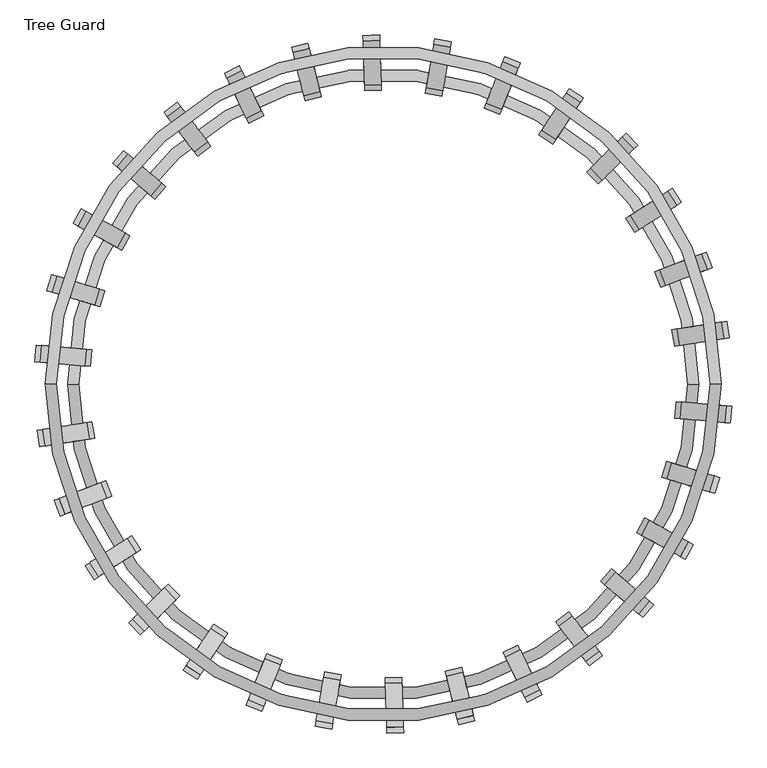
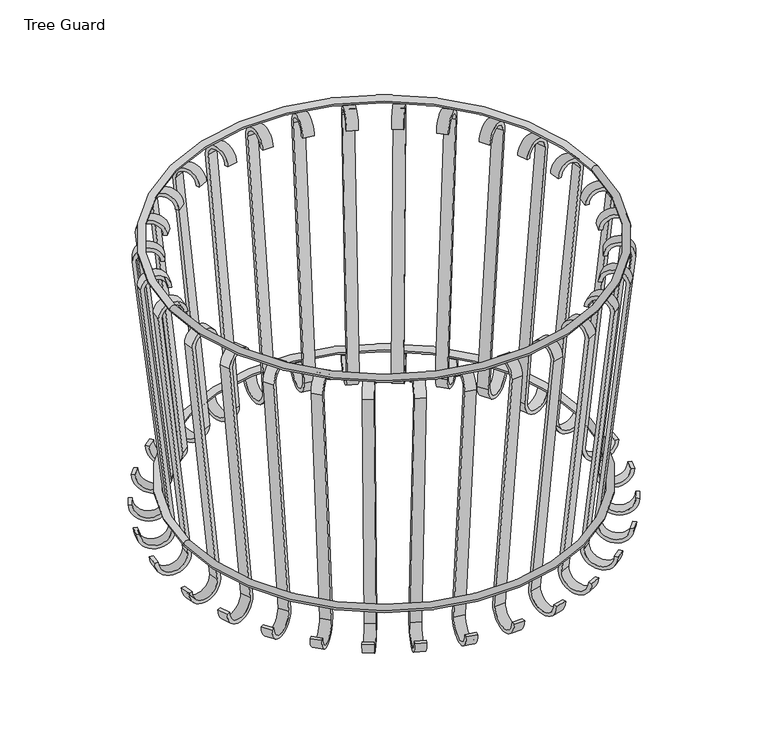
"""IFC4 building model written with IfcOpenShell, lengths in millimetres: railing geometry, Tree Guard."""

from ifc_helpers import new_model, si_unit, point, frame, frame_2d, origin, origin_2d, place, context, project, spatial, polyline, circle_curve, ellipse_curve, trimmed, segment, composite_curve, outline, extrude, source, transform, mapped, element, save
from ifc_brep_helpers import revolved_surface, advanced_brep


def tree_guard_4b5819f2(model_context):
    return source(origin(), model_context, "Body", "SolidModel", [
        advanced_brep(
        [(1686.3981957, 17584.520735, 1003.3), (3235.7981957, 17584.520735, 1003.3), (3210.3981957, 17584.520735, 1003.3), (1711.7981957, 17584.520735, 1003.3)],
        [
            (0, 1, circle_curve(frame((2461.0981957, 17584.520735, 1003.3), z_axis=(0.0, 0.0, -1.0), x_axis=(1.0, 0.0, 0.0)), 774.7)),
            (1, 2, circle_curve(frame((3223.0981957, 17584.520735, 1003.3), z_axis=(0.0, 1.0, 0.0), x_axis=(-1.0, 0.0, 0.0)), 12.7)),
            (2, 3, circle_curve(frame((2461.0981957, 17584.520735, 1003.3), z_axis=(0.0, 0.0, 1.0), x_axis=(1.0, 0.0, 0.0)), 749.3)),
            (3, 0, circle_curve(frame((1699.0981957, 17584.520735, 1003.3), z_axis=(0.0, 1.0, 0.0), x_axis=(1.0, 0.0, 0.0)), 12.7)),
            (2, 1, circle_curve(frame((3223.0981957, 17584.520735, 1003.3), z_axis=(0.0, 1.0, 0.0), x_axis=(-1.0, 0.0, 0.0)), 12.7)),
            (0, 3, circle_curve(frame((1699.0981957, 17584.520735, 1003.3), z_axis=(0.0, 1.0, 0.0), x_axis=(1.0, 0.0, 0.0)), 12.7)),
            (1, 0, circle_curve(frame((2461.0981957, 17584.520735, 1003.3), z_axis=(0.0, 0.0, -1.0), x_axis=(-1.0, 0.0, 0.0)), 774.7)),
            (3, 2, circle_curve(frame((2461.0981957, 17584.520735, 1003.3), z_axis=(0.0, 0.0, 1.0), x_axis=(-1.0, 0.0, 0.0)), 749.3)),
        ],
        [
            revolved_surface(trimmed(ellipse_curve(frame((3223.0981957, 17584.520735, 1003.3), z_axis=(0.0, -1.0, 0.0), x_axis=(-1.0, 0.0, 0.0)), 12.7, 12.7), [point((3210.3981957, 17584.520735, 1003.3))], [point((3235.7981957, 17584.520735, 1003.3))], True, "CARTESIAN"), (2461.0981957, 17584.520735, 1016.0), (0.0, 0.0, 1.0)),
            revolved_surface(trimmed(ellipse_curve(frame((3223.0981957, 17584.520735, 1003.3), z_axis=(0.0, -1.0, 0.0), x_axis=(-1.0, 0.0, 0.0)), 12.7, 12.7), [point((3235.7981957, 17584.520735, 1003.3))], [point((3210.3981957, 17584.520735, 1003.3))], True, "CARTESIAN"), (2461.0981957, 17584.520735, 1016.0), (0.0, 0.0, 1.0)),
            revolved_surface(trimmed(ellipse_curve(frame((1699.0981957, 17584.520735, 1003.3), z_axis=(0.0, 1.0, 0.0), x_axis=(1.0, 0.0, 0.0)), 12.7, 12.7), [point((1711.7981957, 17584.520735, 1003.3))], [point((1686.3981957, 17584.520735, 1003.3))], True, "CARTESIAN"), (2461.0981957, 17584.520735, 1016.0), (0.0, 0.0, 1.0)),
            revolved_surface(trimmed(ellipse_curve(frame((1699.0981957, 17584.520735, 1003.3), z_axis=(0.0, 1.0, 0.0), x_axis=(1.0, 0.0, 0.0)), 12.7, 12.7), [point((1686.3981957, 17584.520735, 1003.3))], [point((1711.7981957, 17584.520735, 1003.3))], True, "CARTESIAN"), (2461.0981957, 17584.520735, 1016.0), (0.0, 0.0, 1.0)),
        ],
        [
            (0, [[1, 2, 3, 4]]),
            (1, [[-3, 5, -1, 6]]),
            (2, [[7, -4, 8, -2]]),
            (3, [[-8, -6, -7, -5]]),
        ],
    ),
        advanced_brep(
        [(1737.1981957, 17584.520735, 88.9), (3184.9981957, 17584.520735, 88.9), (3159.5981957, 17584.520735, 88.9), (1762.5981957, 17584.520735, 88.9)],
        [
            (0, 1, circle_curve(frame((2461.0981957, 17584.520735, 88.9), z_axis=(0.0, 0.0, -1.0), x_axis=(1.0, 0.0, 0.0)), 723.9)),
            (1, 2, circle_curve(frame((3172.2981957, 17584.520735, 88.9), z_axis=(0.0, 1.0, 0.0), x_axis=(-1.0, 0.0, 0.0)), 12.7)),
            (2, 3, circle_curve(frame((2461.0981957, 17584.520735, 88.9), z_axis=(0.0, 0.0, 1.0), x_axis=(1.0, 0.0, 0.0)), 698.5)),
            (3, 0, circle_curve(frame((1749.8981957, 17584.520735, 88.9), z_axis=(0.0, 1.0, 0.0), x_axis=(1.0, 0.0, 0.0)), 12.7)),
            (2, 1, circle_curve(frame((3172.2981957, 17584.520735, 88.9), z_axis=(0.0, 1.0, 0.0), x_axis=(-1.0, 0.0, 0.0)), 12.7)),
            (0, 3, circle_curve(frame((1749.8981957, 17584.520735, 88.9), z_axis=(0.0, 1.0, 0.0), x_axis=(1.0, 0.0, 0.0)), 12.7)),
            (1, 0, circle_curve(frame((2461.0981957, 17584.520735, 88.9), z_axis=(0.0, 0.0, -1.0), x_axis=(-1.0, 0.0, 0.0)), 723.9)),
            (3, 2, circle_curve(frame((2461.0981957, 17584.520735, 88.9), z_axis=(0.0, 0.0, 1.0), x_axis=(-1.0, 0.0, 0.0)), 698.5)),
        ],
        [
            revolved_surface(trimmed(ellipse_curve(frame((3172.2981957, 17584.520735, 88.9), z_axis=(0.0, -1.0, 0.0), x_axis=(-1.0, 0.0, 0.0)), 12.7, 12.7), [point((3159.5981957, 17584.520735, 88.9))], [point((3184.9981957, 17584.520735, 88.9))], True, "CARTESIAN"), (2461.0981957, 17584.520735, 101.6), (0.0, 0.0, 1.0)),
            revolved_surface(trimmed(ellipse_curve(frame((3172.2981957, 17584.520735, 88.9), z_axis=(0.0, -1.0, 0.0), x_axis=(-1.0, 0.0, 0.0)), 12.7, 12.7), [point((3184.9981957, 17584.520735, 88.9))], [point((3159.5981957, 17584.520735, 88.9))], True, "CARTESIAN"), (2461.0981957, 17584.520735, 101.6), (0.0, 0.0, 1.0)),
            revolved_surface(trimmed(ellipse_curve(frame((1749.8981957, 17584.520735, 88.9), z_axis=(0.0, 1.0, 0.0), x_axis=(1.0, 0.0, 0.0)), 12.7, 12.7), [point((1762.5981957, 17584.520735, 88.9))], [point((1737.1981957, 17584.520735, 88.9))], True, "CARTESIAN"), (2461.0981957, 17584.520735, 101.6), (0.0, 0.0, 1.0)),
            revolved_surface(trimmed(ellipse_curve(frame((1749.8981957, 17584.520735, 88.9), z_axis=(0.0, 1.0, 0.0), x_axis=(1.0, 0.0, 0.0)), 12.7, 12.7), [point((1737.1981957, 17584.520735, 88.9))], [point((1762.5981957, 17584.520735, 88.9))], True, "CARTESIAN"), (2461.0981957, 17584.520735, 101.6), (0.0, 0.0, 1.0)),
        ],
        [
            (0, [[1, 2, 3, 4]]),
            (1, [[-3, 5, -1, 6]]),
            (2, [[7, -4, 8, -2]]),
            (3, [[-8, -6, -7, -5]]),
        ],
    ),
        extrude(outline(composite_curve([segment(polyline([(-50.8, 0.0), (-38.1, 0.0)]), True, "CONTINUOUS"), segment(trimmed(circle_curve(origin_2d(), 38.1), [point((-38.1, 0.0))], [point((38.0945547, -0.6441257))], True, "CARTESIAN"), True, "CONTINUOUS"), segment(polyline([(38.0945547, -0.6441257), (-63.4957767, 926.3676491)]), True, "CONTINUOUS"), segment(trimmed(circle_curve(frame_2d((0.0, 927.1)), 63.5), [point((-63.4957767, 926.3676491))], [point((63.5000001, 927.1))], False, "CARTESIAN"), True, "CONTINUOUS"), segment(polyline([(63.5000001, 927.1), (50.8, 927.1)]), True, "CONTINUOUS"), segment(trimmed(circle_curve(frame_2d((0.0, 927.1)), 50.8), [point((50.8, 927.1))], [point((-50.8, 927.1))], True, "CARTESIAN"), True, "CONTINUOUS"), segment(polyline([(-50.8, 927.1), (50.8, 0.0)]), True, "CONTINUOUS"), segment(trimmed(circle_curve(origin_2d(), 50.8), [point((50.8, 0.0))], [point((-50.8, 0.0))], False, "CARTESIAN"), True, "CONTINUOUS")], self_intersect=False)), frame((3193.1705264, 17500.7796751, 939.8), z_axis=(0.08792402544180011, 0.9961271835213162, 0.0), x_axis=(0.996127183521316, -0.0879240254418001, 0.0)), (0.0, 0.0, 1.0), 38.1),
        extrude(outline(composite_curve([segment(polyline([(-50.8000001, 0.0), (-38.1, 0.0)]), True, "CONTINUOUS"), segment(trimmed(circle_curve(origin_2d(), 38.1), [point((-38.1, 0.0))], [point((38.0945547, -0.6441257))], True, "CARTESIAN"), True, "CONTINUOUS"), segment(polyline([(38.0945547, -0.6441257), (-63.4957768, 926.3676491)]), True, "CONTINUOUS"), segment(trimmed(circle_curve(frame_2d((0.0, 927.1)), 63.5), [point((-63.4957768, 926.3676491))], [point((63.5, 927.1))], False, "CARTESIAN"), True, "CONTINUOUS"), segment(polyline([(63.5, 927.1), (50.8, 927.1)]), True, "CONTINUOUS"), segment(trimmed(circle_curve(frame_2d((0.0, 927.1)), 50.8), [point((50.8, 927.1))], [point((-50.8000001, 927.1))], True, "CARTESIAN"), True, "CONTINUOUS"), segment(polyline([(-50.8000001, 927.1), (50.8, 0.0)]), True, "CONTINUOUS"), segment(trimmed(circle_curve(origin_2d(), 50.8), [point((50.8, 0.0))], [point((-50.8000001, 0.0))], False, "CARTESIAN"), True, "CONTINUOUS")], self_intersect=False)), frame((3160.3553357, 17352.1806508, 939.8), z_axis=(0.2906769472457086, 0.9568212541221666, 0.0), x_axis=(0.9568212541221666, -0.2906769472457086, 0.0)), (0.0, 0.0, 1.0), 38.1),
        extrude(outline(composite_curve([segment(polyline([(-50.8000001, 0.0), (-38.1000001, 0.0)]), True, "CONTINUOUS"), segment(trimmed(circle_curve(origin_2d(), 38.1), [point((-38.1000001, 0.0))], [point((38.0945547, -0.6441257))], True, "CARTESIAN"), True, "CONTINUOUS"), segment(polyline([(38.0945547, -0.6441257), (-63.4957768, 926.3676491)]), True, "CONTINUOUS"), segment(trimmed(circle_curve(frame_2d((0.0, 927.1)), 63.5), [point((-63.4957768, 926.3676491))], [point((63.5, 927.1))], False, "CARTESIAN"), True, "CONTINUOUS"), segment(polyline([(63.5, 927.1), (50.8, 927.1)]), True, "CONTINUOUS"), segment(trimmed(circle_curve(frame_2d((0.0, 927.1)), 50.8), [point((50.8, 927.1))], [point((-50.8000001, 927.1))], True, "CARTESIAN"), True, "CONTINUOUS"), segment(polyline([(-50.8000001, 927.1), (50.8, 0.0)]), True, "CONTINUOUS"), segment(trimmed(circle_curve(origin_2d(), 50.8), [point((50.8, 0.0))], [point((-50.8000001, 0.0))], False, "CARTESIAN"), True, "CONTINUOUS")], self_intersect=False)), frame((3097.7142383, 17213.4917916, 939.8), z_axis=(0.48103142076066435, 0.8767033547563148, 0.0), x_axis=(0.8767033547563148, -0.48103142076066435, 0.0)), (0.0, 0.0, 1.0), 38.1),
        extrude(outline(composite_curve([segment(polyline([(-50.8, 0.0), (-38.1, 0.0)]), True, "CONTINUOUS"), segment(trimmed(circle_curve(origin_2d(), 38.1), [point((-38.1, 0.0))], [point((38.0945547, -0.6441257))], True, "CARTESIAN"), True, "CONTINUOUS"), segment(polyline([(38.0945547, -0.6441257), (-63.4957767, 926.3676491)]), True, "CONTINUOUS"), segment(trimmed(circle_curve(frame_2d((0.0, 927.1)), 63.5), [point((-63.4957767, 926.3676491))], [point((63.5, 927.1))], False, "CARTESIAN"), True, "CONTINUOUS"), segment(polyline([(63.5, 927.1), (50.8, 927.1)]), True, "CONTINUOUS"), segment(trimmed(circle_curve(frame_2d((0.0, 927.1)), 50.8), [point((50.8, 927.1))], [point((-50.8, 927.1))], True, "CARTESIAN"), True, "CONTINUOUS"), segment(polyline([(-50.8, 927.1), (50.8, 0.0)]), True, "CONTINUOUS"), segment(trimmed(circle_curve(origin_2d(), 50.8), [point((50.8, 0.0))], [point((-50.8, 0.0))], False, "CARTESIAN"), True, "CONTINUOUS")], self_intersect=False)), frame((3007.919109, 17090.6286909, 939.8), z_axis=(0.6508681227351707, 0.7591908105392182, 0.0), x_axis=(0.759190810539218, -0.6508681227351706, 0.0)), (0.0, 0.0, 1.0), 38.1),
        extrude(outline(composite_curve([segment(polyline([(-50.8, 0.0), (-38.1, 0.0)]), True, "CONTINUOUS"), segment(trimmed(circle_curve(origin_2d(), 38.1), [point((-38.1, 0.0))], [point((38.0945548, -0.6441257))], True, "CARTESIAN"), True, "CONTINUOUS"), segment(polyline([(38.0945548, -0.6441257), (-63.4957767, 926.3676491)]), True, "CONTINUOUS"), segment(trimmed(circle_curve(frame_2d((0.0, 927.1)), 63.5), [point((-63.4957767, 926.3676491))], [point((63.5, 927.1))], False, "CARTESIAN"), True, "CONTINUOUS"), segment(polyline([(63.5, 927.1), (50.8, 927.1)]), True, "CONTINUOUS"), segment(trimmed(circle_curve(frame_2d((0.0, 927.1)), 50.8), [point((50.8, 927.1))], [point((-50.8, 927.1))], True, "CARTESIAN"), True, "CONTINUOUS"), segment(polyline([(-50.8, 927.1), (50.8, 0.0)]), True, "CONTINUOUS"), segment(trimmed(circle_curve(origin_2d(), 50.8), [point((50.8, 0.0))], [point((-50.8, 0.0))], False, "CARTESIAN"), True, "CONTINUOUS")], self_intersect=False)), frame((2894.8000427, 16988.8319149, 939.8), z_axis=(0.7929428888591603, 0.6092959666760394, 0.0), x_axis=(0.6092959666760394, -0.7929428888591603, 0.0)), (0.0, 0.0, 1.0), 38.1),
        extrude(outline(composite_curve([segment(polyline([(-50.8, 0.0), (-38.1000001, 0.0)]), True, "CONTINUOUS"), segment(trimmed(circle_curve(origin_2d(), 38.1), [point((-38.1000001, 0.0))], [point((38.0945548, -0.6441257))], True, "CARTESIAN"), True, "CONTINUOUS"), segment(polyline([(38.0945548, -0.6441257), (-63.4957768, 926.3676491)]), True, "CONTINUOUS"), segment(trimmed(circle_curve(frame_2d((0.0, 927.1)), 63.5), [point((-63.4957768, 926.3676491))], [point((63.5, 927.1))], False, "CARTESIAN"), True, "CONTINUOUS"), segment(polyline([(63.5, 927.1), (50.7999999, 927.1)]), True, "CONTINUOUS"), segment(trimmed(circle_curve(frame_2d((0.0, 927.1)), 50.8), [point((50.7999999, 927.1))], [point((-50.8, 927.1))], True, "CARTESIAN"), True, "CONTINUOUS"), segment(polyline([(-50.8, 927.1), (50.7999999, 0.0)]), True, "CONTINUOUS"), segment(trimmed(circle_curve(origin_2d(), 50.8), [point((50.7999999, 0.0))], [point((-50.8, 0.0))], False, "CARTESIAN"), True, "CONTINUOUS")], self_intersect=False)), frame((2763.1819865, 16912.4434732, 939.8), z_axis=(0.9011957041997504, 0.43341239337600407, 0.0), x_axis=(0.43341239337600407, -0.9011957041997504, 0.0)), (0.0, 0.0, 1.0), 38.1),
        extrude(outline(composite_curve([segment(polyline([(-50.8, 0.0), (-38.1, 0.0)]), True, "CONTINUOUS"), segment(trimmed(circle_curve(origin_2d(), 38.1), [point((-38.1, 0.0))], [point((38.0945548, -0.6441257))], True, "CARTESIAN"), True, "CONTINUOUS"), segment(polyline([(38.0945548, -0.6441257), (-63.4957767, 926.3676491)]), True, "CONTINUOUS"), segment(trimmed(circle_curve(frame_2d((0.0, 927.1)), 63.5), [point((-63.4957767, 926.3676491))], [point((63.5, 927.1))], False, "CARTESIAN"), True, "CONTINUOUS"), segment(polyline([(63.5, 927.1), (50.8, 927.1)]), True, "CONTINUOUS"), segment(trimmed(circle_curve(frame_2d((0.0, 927.1)), 50.8), [point((50.8, 927.1))], [point((-50.8, 927.1))], True, "CARTESIAN"), True, "CONTINUOUS"), segment(polyline([(-50.8, 927.1), (50.8, 0.0)]), True, "CONTINUOUS"), segment(trimmed(circle_curve(origin_2d(), 50.8), [point((50.8, 0.0))], [point((-50.8, 0.0))], False, "CARTESIAN"), True, "CONTINUOUS")], self_intersect=False)), frame((2618.6789379, 16864.7216157, 939.8), z_axis=(0.9710091852807093, 0.23904217640511286, 0.0), x_axis=(0.23904217640511286, -0.9710091852807093, 0.0)), (0.0, 0.0, 1.0), 38.1),
        extrude(outline(composite_curve([segment(polyline([(-50.8, 0.0), (-38.1000001, 0.0)]), True, "CONTINUOUS"), segment(trimmed(circle_curve(origin_2d(), 38.1), [point((-38.1000001, 0.0))], [point((38.0945547, -0.6441257))], True, "CARTESIAN"), True, "CONTINUOUS"), segment(polyline([(38.0945547, -0.6441257), (-63.4957767, 926.3676491)]), True, "CONTINUOUS"), segment(trimmed(circle_curve(frame_2d((0.0, 927.1)), 63.5), [point((-63.4957767, 926.3676491))], [point((63.5, 927.1))], False, "CARTESIAN"), True, "CONTINUOUS"), segment(polyline([(63.5, 927.1), (50.7999999, 927.1)]), True, "CONTINUOUS"), segment(trimmed(circle_curve(frame_2d((0.0, 927.1)), 50.8), [point((50.7999999, 927.1))], [point((-50.8, 927.1))], True, "CARTESIAN"), True, "CONTINUOUS"), segment(polyline([(-50.8, 927.1), (50.7999999, 0.0)]), True, "CONTINUOUS"), segment(trimmed(circle_curve(origin_2d(), 50.8), [point((50.7999999, 0.0))], [point((-50.8, 0.0))], False, "CARTESIAN"), True, "CONTINUOUS")], self_intersect=False)), frame((2467.454487, 16847.7018563, 939.8), z_axis=(0.9994055285876695, 0.034475925345105386, 0.0), x_axis=(0.03447592534510538, -0.9994055285876693, 0.0)), (0.0, 0.0, 1.0), 38.1),
        extrude(outline(composite_curve([segment(polyline([(-38.1, 0.0), (-50.7999999, 0.0)]), True, "CONTINUOUS"), segment(trimmed(circle_curve(origin_2d(), 50.8), [point((-50.7999999, 0.0))], [point((50.8, 0.0))], False, "CARTESIAN"), True, "CONTINUOUS"), segment(polyline([(50.8, 0.0), (-50.7999999, -927.1)]), True, "CONTINUOUS"), segment(trimmed(circle_curve(frame_2d((0.0, -927.1)), 50.8), [point((-50.7999999, -927.1))], [point((50.8, -927.1))], True, "CARTESIAN"), True, "CONTINUOUS"), segment(polyline([(50.8, -927.1), (63.5000001, -927.1)]), True, "CONTINUOUS"), segment(trimmed(circle_curve(frame_2d((0.0, -927.1)), 63.5), [point((63.5000001, -927.1))], [point((-63.4957766, -926.3676491))], False, "CARTESIAN"), True, "CONTINUOUS"), segment(polyline([(-63.4957766, -926.3676491), (38.0945548, 0.6441257)]), True, "CONTINUOUS"), segment(trimmed(circle_curve(origin_2d(), 38.1), [point((38.0945548, 0.6441257))], [point((-38.1, 0.0))], True, "CARTESIAN"), True, "CONTINUOUS")], self_intersect=False)), frame((2353.4940281, 16855.5736824, 939.8), z_axis=(-0.9851735249159695, 0.1715608516085285, 0.0), x_axis=(-0.1715608516085285, -0.9851735249159695, 0.0)), (0.0, 0.0, 1.0), 38.1),
        extrude(outline(composite_curve([segment(polyline([(-38.1000001, 0.0), (-50.8, 0.0)]), True, "CONTINUOUS"), segment(trimmed(circle_curve(origin_2d(), 50.8), [point((-50.8, 0.0))], [point((50.7999999, 0.0))], False, "CARTESIAN"), True, "CONTINUOUS"), segment(polyline([(50.7999999, 0.0), (-50.8, -927.1)]), True, "CONTINUOUS"), segment(trimmed(circle_curve(frame_2d((0.0, -927.1)), 50.8), [point((-50.8, -927.1))], [point((50.7999999, -927.1))], True, "CARTESIAN"), True, "CONTINUOUS"), segment(polyline([(50.7999999, -927.1), (63.4999999, -927.1)]), True, "CONTINUOUS"), segment(trimmed(circle_curve(frame_2d((0.0, -927.1)), 63.5), [point((63.4999999, -927.1))], [point((-63.4957768, -926.3676491))], False, "CARTESIAN"), True, "CONTINUOUS"), segment(polyline([(-63.4957768, -926.3676491), (38.0945547, 0.6441257)]), True, "CONTINUOUS"), segment(trimmed(circle_curve(origin_2d(), 38.1), [point((38.0945547, 0.6441257))], [point((-38.1000001, 0.0))], True, "CARTESIAN"), True, "CONTINUOUS")], self_intersect=False)), frame((2206.0459347, 16893.224267, 939.8), z_axis=(-0.9289202219288105, 0.3702799228850107, 0.0), x_axis=(-0.3702799228850107, -0.9289202219288105, 0.0)), (0.0, 0.0, 1.0), 38.1),
        extrude(outline(composite_curve([segment(polyline([(-38.1, 0.0), (-50.8, 0.0)]), True, "CONTINUOUS"), segment(trimmed(circle_curve(origin_2d(), 50.8), [point((-50.8, 0.0))], [point((50.8, 0.0))], False, "CARTESIAN"), True, "CONTINUOUS"), segment(polyline([(50.8, 0.0), (-50.8, -927.1)]), True, "CONTINUOUS"), segment(trimmed(circle_curve(frame_2d((0.0, -927.1)), 50.8), [point((-50.8, -927.1))], [point((50.8, -927.1))], True, "CARTESIAN"), True, "CONTINUOUS"), segment(polyline([(50.8, -927.1), (63.5, -927.1)]), True, "CONTINUOUS"), segment(trimmed(circle_curve(frame_2d((0.0, -927.1)), 63.5), [point((63.5, -927.1))], [point((-63.4957767, -926.3676491))], False, "CARTESIAN"), True, "CONTINUOUS"), segment(polyline([(-63.4957767, -926.3676491), (38.0945547, 0.6441257)]), True, "CONTINUOUS"), segment(trimmed(circle_curve(origin_2d(), 38.1), [point((38.0945547, 0.6441257))], [point((-38.1, 0.0))], True, "CARTESIAN"), True, "CONTINUOUS")], self_intersect=False)), frame((2069.4767649, 16960.3612062, 939.8), z_axis=(-0.8330450313262865, 0.5532051841609823, 0.0), x_axis=(-0.5532051841609823, -0.8330450313262865, 0.0)), (0.0, 0.0, 1.0), 38.1),
        extrude(outline(composite_curve([segment(polyline([(-38.1000001, 0.0), (-50.8000001, 0.0)]), True, "CONTINUOUS"), segment(trimmed(circle_curve(origin_2d(), 50.8), [point((-50.8000001, 0.0))], [point((50.8, 0.0))], False, "CARTESIAN"), True, "CONTINUOUS"), segment(polyline([(50.8, 0.0), (-50.8000001, -927.1)]), True, "CONTINUOUS"), segment(trimmed(circle_curve(frame_2d((0.0, -927.1)), 50.8), [point((-50.8000001, -927.1))], [point((50.8, -927.1))], True, "CARTESIAN"), True, "CONTINUOUS"), segment(polyline([(50.8, -927.1), (63.5, -927.1)]), True, "CONTINUOUS"), segment(trimmed(circle_curve(frame_2d((0.0, -927.1)), 63.5), [point((63.5, -927.1))], [point((-63.4957767, -926.3676491))], False, "CARTESIAN"), True, "CONTINUOUS"), segment(polyline([(-63.4957767, -926.3676491), (38.0945547, 0.6441257)]), True, "CONTINUOUS"), segment(trimmed(circle_curve(origin_2d(), 38.1), [point((38.0945547, 0.6441257))], [point((-38.1000001, 0.0))], True, "CARTESIAN"), True, "CONTINUOUS")], self_intersect=False)), frame((1949.6116994, 17054.1208608, 939.8), z_axis=(-0.7016373850504294, 0.7125341956001799, 0.0), x_axis=(-0.7125341956001799, -0.7016373850504294, 0.0)), (0.0, 0.0, 1.0), 38.1),
        extrude(outline(composite_curve([segment(polyline([(-38.1, 0.0), (-50.8, 0.0)]), True, "CONTINUOUS"), segment(trimmed(circle_curve(origin_2d(), 50.8), [point((-50.8, 0.0))], [point((50.8, 0.0))], False, "CARTESIAN"), True, "CONTINUOUS"), segment(polyline([(50.8, 0.0), (-50.8, -927.1)]), True, "CONTINUOUS"), segment(trimmed(circle_curve(frame_2d((0.0, -927.1)), 50.8), [point((-50.8, -927.1))], [point((50.8, -927.1))], True, "CARTESIAN"), True, "CONTINUOUS"), segment(polyline([(50.8, -927.1), (63.5, -927.1)]), True, "CONTINUOUS"), segment(trimmed(circle_curve(frame_2d((0.0, -927.1)), 63.5), [point((63.5, -927.1))], [point((-63.4957768, -926.3676491))], False, "CARTESIAN"), True, "CONTINUOUS"), segment(polyline([(-63.4957768, -926.3676491), (38.0945548, 0.6441257)]), True, "CONTINUOUS"), segment(trimmed(circle_curve(origin_2d(), 38.1), [point((38.0945548, 0.6441257))], [point((-38.1, 0.0))], True, "CARTESIAN"), True, "CONTINUOUS")], self_intersect=False)), frame((1851.5634272, 17170.5040343, 939.8), z_axis=(-0.5403023058681354, 0.8414709848078993, 0.0), x_axis=(-0.8414709848078993, -0.5403023058681354, 0.0)), (0.0, 0.0, 1.0), 38.1),
        extrude(outline(composite_curve([segment(polyline([(-38.1, 0.0), (-50.8, 0.0)]), True, "CONTINUOUS"), segment(trimmed(circle_curve(origin_2d(), 50.8), [point((-50.8, 0.0))], [point((50.8000001, 0.0))], False, "CARTESIAN"), True, "CONTINUOUS"), segment(polyline([(50.8000001, 0.0), (-50.8, -927.1)]), True, "CONTINUOUS"), segment(trimmed(circle_curve(frame_2d((0.0, -927.1)), 50.8), [point((-50.8, -927.1))], [point((50.8000001, -927.1))], True, "CARTESIAN"), True, "CONTINUOUS"), segment(polyline([(50.8000001, -927.1), (63.5000001, -927.1)]), True, "CONTINUOUS"), segment(trimmed(circle_curve(frame_2d((0.0, -927.1)), 63.5), [point((63.5000001, -927.1))], [point((-63.4957767, -926.3676491))], False, "CARTESIAN"), True, "CONTINUOUS"), segment(polyline([(-63.4957767, -926.3676491), (38.0945548, 0.6441257)]), True, "CONTINUOUS"), segment(trimmed(circle_curve(origin_2d(), 38.1), [point((38.0945548, 0.6441257))], [point((-38.1, 0.0))], True, "CARTESIAN"), True, "CONTINUOUS")], self_intersect=False)), frame((1779.5140703, 17304.5465533, 939.8), z_axis=(-0.35592133239259605, 0.9345159202217368, 0.0), x_axis=(-0.9345159202217366, -0.355921332392596, 0.0)), (0.0, 0.0, 1.0), 38.1),
        extrude(outline(composite_curve([segment(polyline([(-38.1, 0.0), (-50.8, 0.0)]), True, "CONTINUOUS"), segment(trimmed(circle_curve(origin_2d(), 50.8), [point((-50.8, 0.0))], [point((50.8, 0.0))], False, "CARTESIAN"), True, "CONTINUOUS"), segment(polyline([(50.8, 0.0), (-50.8, -927.1)]), True, "CONTINUOUS"), segment(trimmed(circle_curve(frame_2d((0.0, -927.1)), 50.8), [point((-50.8, -927.1))], [point((50.8, -927.1))], True, "CARTESIAN"), True, "CONTINUOUS"), segment(polyline([(50.8, -927.1), (63.5, -927.1)]), True, "CONTINUOUS"), segment(trimmed(circle_curve(frame_2d((0.0, -927.1)), 63.5), [point((63.5, -927.1))], [point((-63.4957767, -926.3676491))], False, "CARTESIAN"), True, "CONTINUOUS"), segment(polyline([(-63.4957767, -926.3676491), (38.0945548, 0.6441257)]), True, "CONTINUOUS"), segment(trimmed(circle_curve(origin_2d(), 38.1), [point((38.0945548, 0.6441257))], [point((-38.1, 0.0))], True, "CARTESIAN"), True, "CONTINUOUS")], self_intersect=False)), frame((1736.5368004, 17450.5310081, 939.8), z_axis=(-0.15635899597645012, 0.9877002907649852, 0.0), x_axis=(-0.9877002907649852, -0.15635899597645012, 0.0)), (0.0, 0.0, 1.0), 38.1),
        extrude(outline(composite_curve([segment(polyline([(-38.1, 0.0), (-50.8000001, 0.0)]), True, "CONTINUOUS"), segment(trimmed(circle_curve(origin_2d(), 50.8), [point((-50.8000001, 0.0))], [point((50.8, 0.0))], False, "CARTESIAN"), True, "CONTINUOUS"), segment(polyline([(50.8, 0.0), (-50.8000001, -927.1)]), True, "CONTINUOUS"), segment(trimmed(circle_curve(frame_2d((0.0, -927.1)), 50.8), [point((-50.8000001, -927.1))], [point((50.8, -927.1))], True, "CARTESIAN"), True, "CONTINUOUS"), segment(polyline([(50.8, -927.1), (63.5, -927.1)]), True, "CONTINUOUS"), segment(trimmed(circle_curve(frame_2d((0.0, -927.1)), 63.5), [point((63.5, -927.1))], [point((-63.4957768, -926.3676491))], False, "CARTESIAN"), True, "CONTINUOUS"), segment(polyline([(-63.4957768, -926.3676491), (38.0945547, 0.6441257)]), True, "CONTINUOUS"), segment(trimmed(circle_curve(origin_2d(), 38.1), [point((38.0945547, 0.6441257))], [point((-38.1, 0.0))], True, "CARTESIAN"), True, "CONTINUOUS")], self_intersect=False)), frame((1725.6759596, 17630.3093493, 939.8), z_axis=(0.08792402544179688, 0.9961271835213164, 0.0), x_axis=(-0.9961271835213164, 0.08792402544179688, 0.0)), (0.0, 0.0, 1.0), 38.1),
        extrude(outline(composite_curve([segment(polyline([(-38.1, 0.0), (-50.8, 0.0)]), True, "CONTINUOUS"), segment(trimmed(circle_curve(origin_2d(), 50.8), [point((-50.8, 0.0))], [point((50.8, 0.0))], False, "CARTESIAN"), True, "CONTINUOUS"), segment(polyline([(50.8, 0.0), (-50.8, -927.1)]), True, "CONTINUOUS"), segment(trimmed(circle_curve(frame_2d((0.0, -927.1)), 50.8), [point((-50.8, -927.1))], [point((50.8, -927.1))], True, "CARTESIAN"), True, "CONTINUOUS"), segment(polyline([(50.8, -927.1), (63.5, -927.1)]), True, "CONTINUOUS"), segment(trimmed(circle_curve(frame_2d((0.0, -927.1)), 63.5), [point((63.5, -927.1))], [point((-63.4957767, -926.3676491))], False, "CARTESIAN"), True, "CONTINUOUS"), segment(polyline([(-63.4957767, -926.3676491), (38.0945548, 0.6441257)]), True, "CONTINUOUS"), segment(trimmed(circle_curve(origin_2d(), 38.1), [point((38.0945548, 0.6441257))], [point((-38.1, 0.0))], True, "CARTESIAN"), True, "CONTINUOUS")], self_intersect=False)), frame((1750.7662641, 17780.4059295, 939.8), z_axis=(0.2906769472457055, 0.9568212541221675, 0.0), x_axis=(-0.9568212541221675, 0.2906769472457055, 0.0)), (0.0, 0.0, 1.0), 38.1),
        extrude(outline(composite_curve([segment(polyline([(-38.1, 0.0), (-50.8000001, 0.0)]), True, "CONTINUOUS"), segment(trimmed(circle_curve(origin_2d(), 50.8), [point((-50.8000001, 0.0))], [point((50.7999999, 0.0))], False, "CARTESIAN"), True, "CONTINUOUS"), segment(polyline([(50.7999999, 0.0), (-50.8000001, -927.1)]), True, "CONTINUOUS"), segment(trimmed(circle_curve(frame_2d((0.0, -927.1)), 50.8), [point((-50.8000001, -927.1))], [point((50.7999999, -927.1))], True, "CARTESIAN"), True, "CONTINUOUS"), segment(polyline([(50.7999999, -927.1), (63.5, -927.1)]), True, "CONTINUOUS"), segment(trimmed(circle_curve(frame_2d((0.0, -927.1)), 63.5), [point((63.5, -927.1))], [point((-63.4957768, -926.3676491))], False, "CARTESIAN"), True, "CONTINUOUS"), segment(polyline([(-63.4957768, -926.3676491), (38.0945547, 0.6441257)]), True, "CONTINUOUS"), segment(trimmed(circle_curve(origin_2d(), 38.1), [point((38.0945547, 0.6441257))], [point((-38.1, 0.0))], True, "CARTESIAN"), True, "CONTINUOUS")], self_intersect=False)), frame((1806.154856, 17922.1472807, 939.8), z_axis=(0.4810314207606615, 0.8767033547563163, 0.0), x_axis=(-0.8767033547563163, 0.4810314207606615, 0.0)), (0.0, 0.0, 1.0), 38.1),
        extrude(outline(composite_curve([segment(polyline([(-38.1, 0.0), (-50.8, 0.0)]), True, "CONTINUOUS"), segment(trimmed(circle_curve(origin_2d(), 50.8), [point((-50.8, 0.0))], [point((50.7999999, 0.0))], False, "CARTESIAN"), True, "CONTINUOUS"), segment(polyline([(50.7999999, 0.0), (-50.8, -927.1)]), True, "CONTINUOUS"), segment(trimmed(circle_curve(frame_2d((0.0, -927.1)), 50.8), [point((-50.8, -927.1))], [point((50.7999999, -927.1))], True, "CARTESIAN"), True, "CONTINUOUS"), segment(polyline([(50.7999999, -927.1), (63.5, -927.1)]), True, "CONTINUOUS"), segment(trimmed(circle_curve(frame_2d((0.0, -927.1)), 63.5), [point((63.5, -927.1))], [point((-63.4957767, -926.3676491))], False, "CARTESIAN"), True, "CONTINUOUS"), segment(polyline([(-63.4957767, -926.3676491), (38.0945548, 0.6441257)]), True, "CONTINUOUS"), segment(trimmed(circle_curve(origin_2d(), 38.1), [point((38.0945548, 0.6441257))], [point((-38.1, 0.0))], True, "CARTESIAN"), True, "CONTINUOUS")], self_intersect=False)), frame((1889.4792069, 18049.4876093, 939.8), z_axis=(0.6508681227351685, 0.7591908105392199, 0.0), x_axis=(-0.7591908105392199, 0.6508681227351685, 0.0)), (0.0, 0.0, 1.0), 38.1),
        extrude(outline(composite_curve([segment(polyline([(-38.1, 0.0), (-50.8, 0.0)]), True, "CONTINUOUS"), segment(trimmed(circle_curve(origin_2d(), 50.8), [point((-50.8, 0.0))], [point((50.8, 0.0))], False, "CARTESIAN"), True, "CONTINUOUS"), segment(polyline([(50.8, 0.0), (-50.8, -927.1)]), True, "CONTINUOUS"), segment(trimmed(circle_curve(frame_2d((0.0, -927.1)), 50.8), [point((-50.8, -927.1))], [point((50.8, -927.1))], True, "CARTESIAN"), True, "CONTINUOUS"), segment(polyline([(50.8, -927.1), (63.5000001, -927.1)]), True, "CONTINUOUS"), segment(trimmed(circle_curve(frame_2d((0.0, -927.1)), 63.5), [point((63.5000001, -927.1))], [point((-63.4957767, -926.3676491))], False, "CARTESIAN"), True, "CONTINUOUS"), segment(polyline([(-63.4957767, -926.3676491), (38.0945547, 0.6441257)]), True, "CONTINUOUS"), segment(trimmed(circle_curve(origin_2d(), 38.1), [point((38.0945547, 0.6441257))], [point((-38.1, 0.0))], True, "CARTESIAN"), True, "CONTINUOUS")], self_intersect=False)), frame((1997.1852246, 18156.9953788, 939.8), z_axis=(0.7929428888591584, 0.6092959666760419, 0.0), x_axis=(-0.6092959666760419, 0.7929428888591584, 0.0)), (0.0, 0.0, 1.0), 38.1),
        extrude(outline(composite_curve([segment(polyline([(-38.1000001, 0.0), (-50.8, 0.0)]), True, "CONTINUOUS"), segment(trimmed(circle_curve(origin_2d(), 50.8), [point((-50.8, 0.0))], [point((50.7999999, 0.0))], False, "CARTESIAN"), True, "CONTINUOUS"), segment(polyline([(50.7999999, 0.0), (-50.8, -927.1)]), True, "CONTINUOUS"), segment(trimmed(circle_curve(frame_2d((0.0, -927.1)), 50.8), [point((-50.8, -927.1))], [point((50.7999999, -927.1))], True, "CARTESIAN"), True, "CONTINUOUS"), segment(polyline([(50.7999999, -927.1), (63.5, -927.1)]), True, "CONTINUOUS"), segment(trimmed(circle_curve(frame_2d((0.0, -927.1)), 63.5), [point((63.5, -927.1))], [point((-63.4957768, -926.3676491))], False, "CARTESIAN"), True, "CONTINUOUS"), segment(polyline([(-63.4957768, -926.3676491), (38.0945548, 0.6441257)]), True, "CONTINUOUS"), segment(trimmed(circle_curve(origin_2d(), 38.1), [point((38.0945548, 0.6441257))], [point((-38.1000001, 0.0))], True, "CARTESIAN"), True, "CONTINUOUS")], self_intersect=False)), frame((2124.6788486, 18240.0849847, 939.8), z_axis=(0.9011957041997489, 0.433412393376007, 0.0), x_axis=(-0.433412393376007, 0.9011957041997489, 0.0)), (0.0, 0.0, 1.0), 38.1),
        extrude(outline(composite_curve([segment(polyline([(-38.1, 0.0), (-50.8, 0.0)]), True, "CONTINUOUS"), segment(trimmed(circle_curve(origin_2d(), 50.8), [point((-50.8, 0.0))], [point((50.8, 0.0))], False, "CARTESIAN"), True, "CONTINUOUS"), segment(polyline([(50.8, 0.0), (-50.8, -927.1)]), True, "CONTINUOUS"), segment(trimmed(circle_curve(frame_2d((0.0, -927.1)), 50.8), [point((-50.8, -927.1))], [point((50.8, -927.1))], True, "CARTESIAN"), True, "CONTINUOUS"), segment(polyline([(50.8, -927.1), (63.4999999, -927.1)]), True, "CONTINUOUS"), segment(trimmed(circle_curve(frame_2d((0.0, -927.1)), 63.5), [point((63.4999999, -927.1))], [point((-63.4957768, -926.3676491))], False, "CARTESIAN"), True, "CONTINUOUS"), segment(polyline([(-63.4957768, -926.3676491), (38.0945547, 0.6441257)]), True, "CONTINUOUS"), segment(trimmed(circle_curve(origin_2d(), 38.1), [point((38.0945547, 0.6441257))], [point((-38.1, 0.0))], True, "CARTESIAN"), True, "CONTINUOUS")], self_intersect=False)), frame((2266.5220036, 18295.2123475, 939.8), z_axis=(0.9710091852807086, 0.239042176405116, 0.0), x_axis=(-0.239042176405116, 0.9710091852807086, 0.0)), (0.0, 0.0, 1.0), 38.1),
        extrude(outline(composite_curve([segment(polyline([(-38.1, 0.0), (-50.7999999, 0.0)]), True, "CONTINUOUS"), segment(trimmed(circle_curve(origin_2d(), 50.8), [point((-50.7999999, 0.0))], [point((50.8, 0.0))], False, "CARTESIAN"), True, "CONTINUOUS"), segment(polyline([(50.8, 0.0), (-50.7999999, -927.1)]), True, "CONTINUOUS"), segment(trimmed(circle_curve(frame_2d((0.0, -927.1)), 50.8), [point((-50.7999999, -927.1))], [point((50.8, -927.1))], True, "CARTESIAN"), True, "CONTINUOUS"), segment(polyline([(50.8, -927.1), (63.5, -927.1)]), True, "CONTINUOUS"), segment(trimmed(circle_curve(frame_2d((0.0, -927.1)), 63.5), [point((63.5, -927.1))], [point((-63.4957767, -926.3676491))], False, "CARTESIAN"), True, "CONTINUOUS"), segment(polyline([(-63.4957767, -926.3676491), (38.0945548, 0.6441257)]), True, "CONTINUOUS"), segment(trimmed(circle_curve(origin_2d(), 38.1), [point((38.0945548, 0.6441257))], [point((-38.1, 0.0))], True, "CARTESIAN"), True, "CONTINUOUS")], self_intersect=False)), frame((2416.6645538, 18320.026081, 939.8), z_axis=(0.9994055285876694, 0.03447592534510861, 0.0), x_axis=(-0.034475925345108606, 0.9994055285876692, 0.0)), (0.0, 0.0, 1.0), 38.1),
        extrude(outline(composite_curve([segment(polyline([(-50.8, 0.0), (-38.1, 0.0)]), True, "CONTINUOUS"), segment(trimmed(circle_curve(origin_2d(), 38.1), [point((-38.1, 0.0))], [point((38.0945548, -0.6441257))], True, "CARTESIAN"), True, "CONTINUOUS"), segment(polyline([(38.0945548, -0.6441257), (-63.4957768, 926.3676491)]), True, "CONTINUOUS"), segment(trimmed(circle_curve(frame_2d((0.0, 927.1)), 63.5), [point((-63.4957768, 926.3676491))], [point((63.5, 927.1))], False, "CARTESIAN"), True, "CONTINUOUS"), segment(polyline([(63.5, 927.1), (50.7999999, 927.1)]), True, "CONTINUOUS"), segment(trimmed(circle_curve(frame_2d((0.0, 927.1)), 50.8), [point((50.7999999, 927.1))], [point((-50.8, 927.1))], True, "CARTESIAN"), True, "CONTINUOUS"), segment(polyline([(-50.8, 927.1), (50.7999999, 0.0)]), True, "CONTINUOUS"), segment(trimmed(circle_curve(origin_2d(), 50.8), [point((50.7999999, 0.0))], [point((-50.8, 0.0))], False, "CARTESIAN"), True, "CONTINUOUS")], self_intersect=False)), frame((2606.2374747, 18306.9313193, 939.8), z_axis=(-0.9851735249159701, 0.1715608516085253, 0.0), x_axis=(0.1715608516085253, 0.9851735249159701, 0.0)), (0.0, 0.0, 1.0), 38.1),
        extrude(outline(composite_curve([segment(polyline([(-50.8, 0.0), (-38.1, 0.0)]), True, "CONTINUOUS"), segment(trimmed(circle_curve(origin_2d(), 38.1), [point((-38.1, 0.0))], [point((38.0945547, -0.6441257))], True, "CARTESIAN"), True, "CONTINUOUS"), segment(polyline([(38.0945547, -0.6441257), (-63.4957767, 926.3676491)]), True, "CONTINUOUS"), segment(trimmed(circle_curve(frame_2d((0.0, 927.1)), 63.5), [point((-63.4957767, 926.3676491))], [point((63.5, 927.1))], False, "CARTESIAN"), True, "CONTINUOUS"), segment(polyline([(63.5, 927.1), (50.8, 927.1)]), True, "CONTINUOUS"), segment(trimmed(circle_curve(frame_2d((0.0, 927.1)), 50.8), [point((50.8, 927.1))], [point((-50.8, 927.1))], True, "CARTESIAN"), True, "CONTINUOUS"), segment(polyline([(-50.8, 927.1), (50.8, 0.0)]), True, "CONTINUOUS"), segment(trimmed(circle_curve(origin_2d(), 50.8), [point((50.8, 0.0))], [point((-50.8, 0.0))], False, "CARTESIAN"), True, "CONTINUOUS")], self_intersect=False)), frame((2751.5423171, 18261.709538, 939.8), z_axis=(-0.9289202219288119, 0.3702799228850078, 0.0), x_axis=(0.3702799228850077, 0.9289202219288116, 0.0)), (0.0, 0.0, 1.0), 38.1),
        extrude(outline(composite_curve([segment(polyline([(-50.8, 0.0), (-38.1, 0.0)]), True, "CONTINUOUS"), segment(trimmed(circle_curve(origin_2d(), 38.1), [point((-38.1, 0.0))], [point((38.0945547, -0.6441257))], True, "CARTESIAN"), True, "CONTINUOUS"), segment(polyline([(38.0945547, -0.6441257), (-63.4957767, 926.3676491)]), True, "CONTINUOUS"), segment(trimmed(circle_curve(frame_2d((0.0, 927.1)), 63.5), [point((-63.4957767, 926.3676491))], [point((63.5, 927.1))], False, "CARTESIAN"), True, "CONTINUOUS"), segment(polyline([(63.5, 927.1), (50.8, 927.1)]), True, "CONTINUOUS"), segment(trimmed(circle_curve(frame_2d((0.0, 927.1)), 50.8), [point((50.8, 927.1))], [point((-50.8, 927.1))], True, "CARTESIAN"), True, "CONTINUOUS"), segment(polyline([(-50.8, 927.1), (50.8, 0.0)]), True, "CONTINUOUS"), segment(trimmed(circle_curve(origin_2d(), 50.8), [point((50.8, 0.0))], [point((-50.8, 0.0))], False, "CARTESIAN"), True, "CONTINUOUS")], self_intersect=False)), frame((2884.4586422, 18187.6031464, 939.8), z_axis=(-0.8330450313262883, 0.5532051841609796, 0.0), x_axis=(0.5532051841609796, 0.8330450313262883, 0.0)), (0.0, 0.0, 1.0), 38.1),
        extrude(outline(composite_curve([segment(polyline([(-50.8, 0.0), (-38.1, 0.0)]), True, "CONTINUOUS"), segment(trimmed(circle_curve(origin_2d(), 38.1), [point((-38.1, 0.0))], [point((38.0945547, -0.6441257))], True, "CARTESIAN"), True, "CONTINUOUS"), segment(polyline([(38.0945547, -0.6441257), (-63.4957767, 926.3676491)]), True, "CONTINUOUS"), segment(trimmed(circle_curve(frame_2d((0.0, 927.1)), 63.5), [point((-63.4957767, 926.3676491))], [point((63.5, 927.1))], False, "CARTESIAN"), True, "CONTINUOUS"), segment(polyline([(63.5, 927.1), (50.8, 927.1)]), True, "CONTINUOUS"), segment(trimmed(circle_curve(frame_2d((0.0, 927.1)), 50.8), [point((50.8, 927.1))], [point((-50.8, 927.1))], True, "CARTESIAN"), True, "CONTINUOUS"), segment(polyline([(-50.8, 927.1), (50.8, 0.0)]), True, "CONTINUOUS"), segment(trimmed(circle_curve(origin_2d(), 50.8), [point((50.8, 0.0))], [point((-50.8, 0.0))], False, "CARTESIAN"), True, "CONTINUOUS")], self_intersect=False)), frame((2999.3170764, 18087.7730564, 939.8), z_axis=(-0.7016373850504317, 0.7125341956001778, 0.0), x_axis=(0.7125341956001777, 0.7016373850504316, 0.0)), (0.0, 0.0, 1.0), 38.1),
        extrude(outline(composite_curve([segment(polyline([(-50.8, 0.0), (-38.1, 0.0)]), True, "CONTINUOUS"), segment(trimmed(circle_curve(origin_2d(), 38.1), [point((-38.1, 0.0))], [point((38.0945548, -0.6441257))], True, "CARTESIAN"), True, "CONTINUOUS"), segment(polyline([(38.0945548, -0.6441257), (-63.4957767, 926.3676491)]), True, "CONTINUOUS"), segment(trimmed(circle_curve(frame_2d((0.0, 927.1)), 63.5), [point((-63.4957767, 926.3676491))], [point((63.5, 927.1))], False, "CARTESIAN"), True, "CONTINUOUS"), segment(polyline([(63.5, 927.1), (50.8, 927.1)]), True, "CONTINUOUS"), segment(trimmed(circle_curve(frame_2d((0.0, 927.1)), 50.8), [point((50.8, 927.1))], [point((-50.8, 927.1))], True, "CARTESIAN"), True, "CONTINUOUS"), segment(polyline([(-50.8, 927.1), (50.8, 0.0)]), True, "CONTINUOUS"), segment(trimmed(circle_curve(origin_2d(), 50.8), [point((50.8, 0.0))], [point((-50.8, 0.0))], False, "CARTESIAN"), True, "CONTINUOUS")], self_intersect=False)), frame((3091.218482, 17966.4773913, 939.8), z_axis=(-0.5403023058681383, 0.8414709848078974, 0.0), x_axis=(0.8414709848078974, 0.5403023058681383, 0.0)), (0.0, 0.0, 1.0), 38.1),
        extrude(outline(composite_curve([segment(polyline([(-50.8, 0.0), (-38.1, 0.0)]), True, "CONTINUOUS"), segment(trimmed(circle_curve(origin_2d(), 38.1), [point((-38.1, 0.0))], [point((38.0945548, -0.6441257))], True, "CARTESIAN"), True, "CONTINUOUS"), segment(polyline([(38.0945548, -0.6441257), (-63.4957767, 926.3676491)]), True, "CONTINUOUS"), segment(trimmed(circle_curve(frame_2d((0.0, 927.1)), 63.5), [point((-63.4957767, 926.3676491))], [point((63.5000001, 927.1))], False, "CARTESIAN"), True, "CONTINUOUS"), segment(polyline([(63.5000001, 927.1), (50.8000001, 927.1)]), True, "CONTINUOUS"), segment(trimmed(circle_curve(frame_2d((0.0, 927.1)), 50.8), [point((50.8000001, 927.1))], [point((-50.8, 927.1))], True, "CARTESIAN"), True, "CONTINUOUS"), segment(polyline([(-50.8, 927.1), (50.8000001, 0.0)]), True, "CONTINUOUS"), segment(trimmed(circle_curve(origin_2d(), 50.8), [point((50.8000001, 0.0))], [point((-50.8, 0.0))], False, "CARTESIAN"), True, "CONTINUOUS")], self_intersect=False)), frame((3156.2429239, 17828.8898602, 939.8), z_axis=(-0.35592133239259927, 0.9345159202217354, 0.0), x_axis=(0.9345159202217354, 0.35592133239259927, 0.0)), (0.0, 0.0, 1.0), 38.1),
        extrude(outline(composite_curve([segment(polyline([(-50.8, 0.0), (-38.1, 0.0)]), True, "CONTINUOUS"), segment(trimmed(circle_curve(origin_2d(), 38.1), [point((-38.1, 0.0))], [point((38.0945548, -0.6441257))], True, "CARTESIAN"), True, "CONTINUOUS"), segment(polyline([(38.0945548, -0.6441257), (-63.4957768, 926.3676491)]), True, "CONTINUOUS"), segment(trimmed(circle_curve(frame_2d((0.0, 927.1)), 63.5), [point((-63.4957768, 926.3676491))], [point((63.4999999, 927.1))], False, "CARTESIAN"), True, "CONTINUOUS"), segment(polyline([(63.4999999, 927.1), (50.7999999, 927.1)]), True, "CONTINUOUS"), segment(trimmed(circle_curve(frame_2d((0.0, 927.1)), 50.8), [point((50.7999999, 927.1))], [point((-50.8, 927.1))], True, "CARTESIAN"), True, "CONTINUOUS"), segment(polyline([(-50.8, 927.1), (50.7999999, 0.0)]), True, "CONTINUOUS"), segment(trimmed(circle_curve(origin_2d(), 50.8), [point((50.7999999, 0.0))], [point((-50.8, 0.0))], False, "CARTESIAN"), True, "CONTINUOUS")], self_intersect=False)), frame((3191.6168688, 17680.8790809, 939.8), z_axis=(-0.15635899597645306, 0.9877002907649848, 0.0), x_axis=(0.9877002907649848, 0.15635899597645306, 0.0)), (0.0, 0.0, 1.0), 38.1),
    ])


if __name__ == "__main__":
    model = new_model("IFC4")
    model_context = context("Model", 3, world=origin())
    ifc_project = project(units=[si_unit("LENGTHUNIT", "METRE", prefix="MILLI")], contexts=[model_context])
    site = spatial("IfcSite", under=ifc_project)
    building = spatial("IfcBuilding", under=site)
    placement = place(None, origin())
    tree_guard_shape = tree_guard_4b5819f2(model_context)
    element("IfcRailing", 1, ObjectType="Tree Guard", at=placement, inside=building, context=model_context, shape_type="MappedRepresentation", body=[
        mapped(tree_guard_shape, transform((0.0, 0.0, 0.0), x_axis=(1.0, 0.0, 0.0), y_axis=(0.0, 1.0, 0.0), z_axis=(0.0, 0.0, 1.0))),
    ])
    save(model, "model.ifc")
